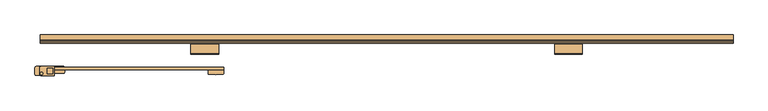
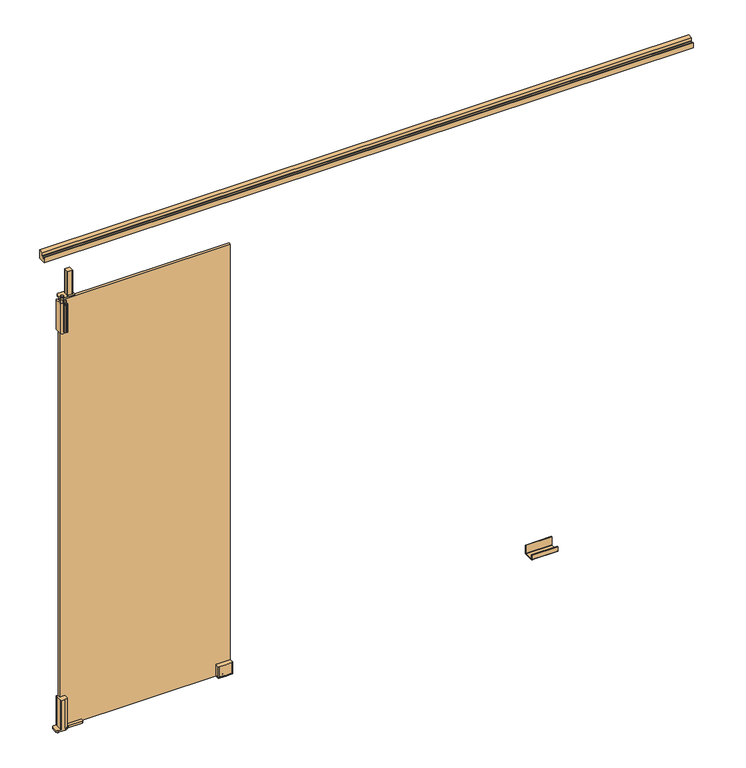
"""IFC4 building model written with IfcOpenShell, lengths in millimetres: door geometry, Otomatik Kapı-Çift Kanat : Otomatik Kapı - Çift Kanat - 150-220."""

from ifc_helpers import new_model, si_unit, point, frame, frame_2d, origin, origin_with_axes, place, context, project, spatial, polyline, circle_curve, trimmed, segment, composite_curve, outline, extrude, source, transform, mapped, element, save
from ifc_brep_helpers import plane_surface, cylinder_surface, revolved_surface, advanced_brep


def door_c3ca8d1c(model_context):
    return source(origin(), model_context, "Body", "SolidModel", [
        advanced_brep(
        [(-1467.3535836, -45.0, 150.5), (-1467.3535836, -42.932554, 150.5), (-1469.2861376, -41.0, 150.5), (-1498.067446, -41.0, 150.5), (-1500.0, -42.932554, 150.5), (-1500.0, -78.2162961, 150.5), (-1498.2162961, -80.0, 150.5), (-1480.406782, -80.0, 150.5), (-1468.0, -73.2159914, 150.5), (-1468.0, -54.9832441, 150.5), (-1493.0, -54.9832441, 150.5), (-1493.0, -45.0, 150.5), (-1471.9265924, -76.964766, 8.0), (-1470.1692976, -75.2261826, 8.0), (-1468.0, -73.2159914, 8.0), (-1493.0, -45.0, 8.0), (-1467.3535836, -45.0, 8.0), (-1493.0, -54.9832441, 8.0), (-1468.0, -54.9832441, 8.0), (-1480.406782, -80.0, 8.0), (-1498.2162961, -80.0, 8.0), (-1512.8478933, -80.0, 8.0), (-1512.8478933, -80.0, 0.0), (-1480.406782, -80.0, 0.0), (-1500.0, -78.2162961, 8.0), (-1500.0, -42.932554, 8.0), (-1498.067446, -41.0, 8.0), (-1469.2861376, -41.0, 8.0), (-1397.0062198, -41.0, 8.0), (-1397.0062198, -41.0, 0.0), (-1512.9502869, -41.0, 0.0), (-1512.9502869, -41.0, 8.0), (-1467.3535836, -42.932554, 8.0), (-1392.0062198, -46.0, 0.0), (-1392.0062198, -66.0, 0.0), (-1397.0062198, -71.0, 0.0), (-1461.1062198, -71.0, 0.0), (-1470.1692976, -75.2261826, 0.0), (-1520.0062198, -72.8416735, 0.0), (-1520.0062198, -48.0559329, 0.0), (-1520.0062198, -48.0559329, 8.0), (-1520.0062198, -72.8416735, 8.0), (-1461.1062198, -71.0, 8.0), (-1397.0062198, -71.0, 8.0), (-1392.0062198, -66.0, 8.0), (-1392.0062198, -46.0, 8.0)],
        [
            (0, 1),
            (1, 2, circle_curve(frame((-1469.2861376, -42.932554, 150.5), z_axis=(0.0, 0.0, 1.0), x_axis=(1.0, 0.0, 0.0)), 1.932554)),
            (2, 3),
            (3, 4, circle_curve(frame((-1498.067446, -42.932554, 150.5), z_axis=(0.0, 0.0, 1.0), x_axis=(1.0, 0.0, 0.0)), 1.932554)),
            (4, 5),
            (5, 6, circle_curve(frame((-1498.2162961, -78.2162961, 150.5), z_axis=(0.0, 0.0, 1.0), x_axis=(1.0, 0.0, 0.0)), 1.7837039)),
            (6, 7),
            (7, 8, circle_curve(frame((-1481.829294, -62.6615339, 150.5), z_axis=(0.0, 0.0, 1.0), x_axis=(1.0, 0.0, 0.0)), 17.3967223)),
            (8, 9),
            (9, 10),
            (10, 11),
            (11, 0),
            (12, 13, circle_curve(frame((-1480.406782, -66.6359132, 8.0), z_axis=(0.0, 0.0, 1.0), x_axis=(1.0, 0.0, 0.0)), 13.3640868)),
            (13, 14, circle_curve(frame((-1461.1062198, -82.8310079, 8.0), z_axis=(0.0, 0.0, -1.0), x_axis=(1.0, 0.0, 0.0)), 11.8310079)),
            (14, 12, circle_curve(frame((-1481.829294, -62.6615339, 8.0), z_axis=(0.0, 0.0, -1.0), x_axis=(1.0, 0.0, 0.0)), 17.3967223)),
            (11, 15),
            (15, 16),
            (16, 0),
            (10, 17),
            (17, 15),
            (9, 18),
            (18, 17),
            (8, 14),
            (14, 18),
            (7, 19),
            (19, 12, circle_curve(frame((-1481.829294, -62.6615339, 8.0), z_axis=(0.0, 0.0, 1.0), x_axis=(1.0, 0.0, 0.0)), 17.3967223)),
            (6, 20),
            (20, 21),
            (21, 22),
            (22, 23),
            (23, 19),
            (5, 24),
            (24, 20, circle_curve(frame((-1498.2162961, -78.2162961, 8.0), z_axis=(0.0, 0.0, 1.0), x_axis=(1.0, 0.0, 0.0)), 1.7837039)),
            (4, 25),
            (25, 24),
            (3, 26),
            (26, 25, circle_curve(frame((-1498.067446, -42.932554, 8.0), z_axis=(0.0, 0.0, 1.0), x_axis=(1.0, 0.0, 0.0)), 1.932554)),
            (2, 27),
            (27, 28),
            (28, 29),
            (29, 30),
            (30, 31),
            (31, 26),
            (1, 32),
            (32, 27, circle_curve(frame((-1469.2861376, -42.932554, 8.0), z_axis=(0.0, 0.0, 1.0), x_axis=(1.0, 0.0, 0.0)), 1.932554)),
            (16, 32),
            (29, 33, circle_curve(frame((-1397.0062198, -46.0, 0.0), z_axis=(0.0, 0.0, -1.0), x_axis=(1.0, 0.0, 0.0)), 5.0)),
            (33, 34),
            (34, 35, circle_curve(frame((-1397.0062198, -66.0, 0.0), z_axis=(0.0, 0.0, -1.0), x_axis=(1.0, 0.0, 0.0)), 5.0)),
            (35, 36),
            (36, 37, circle_curve(frame((-1461.1062198, -82.8310079, 0.0), z_axis=(0.0, 0.0, 1.0), x_axis=(1.0, 0.0, 0.0)), 11.8310079)),
            (37, 23, circle_curve(frame((-1480.406782, -66.6359132, 0.0), z_axis=(0.0, 0.0, -1.0), x_axis=(1.0, 0.0, 0.0)), 13.3640868)),
            (22, 38, circle_curve(frame((-1512.8478933, -72.8416735, 0.0), z_axis=(0.0, 0.0, -1.0), x_axis=(1.0, 0.0, 0.0)), 7.1583265)),
            (38, 39),
            (39, 30, circle_curve(frame((-1512.9502869, -48.0559329, 0.0), z_axis=(0.0, 0.0, -1.0), x_axis=(1.0, 0.0, 0.0)), 7.0559329)),
            (19, 12, circle_curve(frame((-1480.406782, -66.6359132, 8.0), z_axis=(0.0, 0.0, 1.0), x_axis=(1.0, 0.0, 0.0)), 13.3640868)),
            (31, 40, circle_curve(frame((-1512.9502869, -48.0559329, 8.0), z_axis=(0.0, 0.0, 1.0), x_axis=(1.0, 0.0, 0.0)), 7.0559329)),
            (40, 41),
            (41, 21, circle_curve(frame((-1512.8478933, -72.8416735, 8.0), z_axis=(0.0, 0.0, 1.0), x_axis=(1.0, 0.0, 0.0)), 7.1583265)),
            (14, 42, circle_curve(frame((-1461.1062198, -82.8310079, 8.0), z_axis=(0.0, 0.0, -1.0), x_axis=(1.0, 0.0, 0.0)), 11.8310079)),
            (42, 43),
            (43, 44, circle_curve(frame((-1397.0062198, -66.0, 8.0), z_axis=(0.0, 0.0, 1.0), x_axis=(1.0, 0.0, 0.0)), 5.0)),
            (44, 45),
            (45, 28, circle_curve(frame((-1397.0062198, -46.0, 8.0), z_axis=(0.0, 0.0, 1.0), x_axis=(1.0, 0.0, 0.0)), 5.0)),
            (39, 40),
            (38, 41),
            (37, 13),
            (36, 42),
            (35, 43),
            (34, 44),
            (33, 45),
        ],
        [
            plane_surface(frame((-1520.0062198, -41.0, 150.5), z_axis=(0.0, 0.0, 1.0), x_axis=(0.0, 1.0, 0.0))),
            plane_surface(frame((-1520.0062198, -41.0, 8.0), z_axis=(0.0, 0.0, -1.0), x_axis=(0.0, 1.0, 0.0))),
            plane_surface(frame((-1467.3535836, -45.0, 150.5), z_axis=(0.0, -1.0, 0.0), x_axis=(0.0, 0.0, -1.0))),
            plane_surface(frame((-1493.0, -45.0, 150.5), z_axis=(1.0, 0.0, 0.0), x_axis=(0.0, 0.0, -1.0))),
            plane_surface(frame((-1493.0, -54.9832441, 150.5), z_axis=(0.0, 1.0, 0.0), x_axis=(0.0, 0.0, -1.0))),
            plane_surface(frame((-1468.0, -54.9832441, 150.5), z_axis=(1.0, 0.0, 0.0), x_axis=(0.0, 0.0, -1.0))),
            cylinder_surface(frame((-1481.829294, -62.6615339, 150.5), z_axis=(0.0, 0.0, 1.0), x_axis=(1.0, 0.0, 0.0)), 17.3967223),
            plane_surface(frame((-1480.406782, -80.0, 150.5), z_axis=(0.0, -1.0, 0.0), x_axis=(0.0, 0.0, -1.0))),
            cylinder_surface(frame((-1498.2162961, -78.2162961, 150.5), z_axis=(0.0, 0.0, 1.0), x_axis=(1.0, 0.0, 0.0)), 1.7837039),
            plane_surface(frame((-1500.0, -78.2162961, 150.5), z_axis=(-1.0, 0.0, 0.0), x_axis=(0.0, 0.0, -1.0))),
            cylinder_surface(frame((-1498.067446, -42.932554, 150.5), z_axis=(0.0, 0.0, 1.0), x_axis=(1.0, 0.0, 0.0)), 1.932554),
            plane_surface(frame((-1498.067446, -41.0, 150.5), z_axis=(0.0, 1.0, 0.0), x_axis=(0.0, 0.0, -1.0))),
            cylinder_surface(frame((-1469.2861376, -42.932554, 150.5), z_axis=(0.0, 0.0, 1.0), x_axis=(1.0, 0.0, 0.0)), 1.932554),
            plane_surface(frame((-1467.3535836, -42.932554, 150.5), z_axis=(1.0, 0.0, 0.0), x_axis=(0.0, 0.0, -1.0))),
            plane_surface(frame((-1520.0062198, -41.0, 0.0), z_axis=(0.0, 0.0, -1.0), x_axis=(0.0, 1.0, 0.0))),
            plane_surface(frame((-1520.0062198, -41.0, 8.0), z_axis=(0.0, 0.0, 1.0), x_axis=(0.0, 1.0, 0.0))),
            cylinder_surface(frame((-1512.9502869, -48.0559329, 0.0), z_axis=(0.0, 0.0, -1.0), x_axis=(1.0, 0.0, 0.0)), 7.0559329),
            plane_surface(frame((-1520.0062198, -48.0559329, 0.0), z_axis=(-1.0, 0.0, 0.0), x_axis=(0.0, 0.0, 1.0))),
            cylinder_surface(frame((-1512.8478933, -72.8416735, 0.0), z_axis=(0.0, 0.0, -1.0), x_axis=(1.0, 0.0, 0.0)), 7.1583265),
            cylinder_surface(frame((-1480.406782, -66.6359132, 0.0), z_axis=(0.0, 0.0, -1.0), x_axis=(1.0, 0.0, 0.0)), 13.3640868),
            revolved_surface(polyline([(-1449.2752119, -82.8310079, 8.0), (-1449.2752119, -82.8310079, 0.0)]), (-1461.1062198, -82.8310079, 0.0), (0.0, 0.0, 1.0)),
            plane_surface(frame((-1461.1062198, -71.0, 0.0), z_axis=(0.0, -1.0, 0.0), x_axis=(0.0, 0.0, 1.0))),
            cylinder_surface(frame((-1397.0062198, -66.0, 0.0), z_axis=(0.0, 0.0, -1.0), x_axis=(1.0, 0.0, 0.0)), 5.0),
            plane_surface(frame((-1392.0062198, -66.0, 0.0), z_axis=(1.0, 0.0, 0.0), x_axis=(0.0, 0.0, 1.0))),
            cylinder_surface(frame((-1397.0062198, -46.0, 0.0), z_axis=(0.0, 0.0, -1.0), x_axis=(1.0, 0.0, 0.0)), 5.0),
        ],
        [
            (0, [[1, 2, 3, 4, 5, 6, 7, 8, 9, 10, 11, 12]]),
            (1, [[13, 14, 15]]),
            (2, [[16, 17, 18, -12]]),
            (3, [[19, 20, -16, -11]]),
            (4, [[21, 22, -19, -10]]),
            (5, [[23, 24, -21, -9]]),
            (6, [[25, 26, -15, -23, -8]]),
            (7, [[27, 28, 29, 30, 31, -25, -7]]),
            (8, [[32, 33, -27, -6]]),
            (9, [[34, 35, -32, -5]]),
            (10, [[36, 37, -34, -4]]),
            (11, [[38, 39, 40, 41, 42, 43, -36, -3]]),
            (12, [[44, 45, -38, -2]]),
            (13, [[-18, 46, -44, -1]]),
            (14, [[47, 48, 49, 50, 51, 52, -30, 53, 54, 55, -41]]),
            (15, [[-26, 56]]),
            (15, [[-28, -33, -35, -37, -43, 57, 58, 59]]),
            (15, [[-39, -45, -46, -17, -20, -22, -24, 60, 61, 62, 63, 64]]),
            (16, [[65, -57, -42, -55]]),
            (17, [[66, -58, -65, -54]]),
            (18, [[-29, -59, -66, -53]]),
            (19, [[67, -13, -56, -31, -52]]),
            (20, [[68, -60, -14, -67, -51]]),
            (21, [[69, -61, -68, -50]]),
            (22, [[70, -62, -69, -49]]),
            (23, [[71, -63, -70, -48]]),
            (24, [[-40, -64, -71, -47]]),
        ],
    ),
        advanced_brep(
        [(-1465.150075, -48.2790947, 2225.0), (-1466.9853602, -50.1143799, 2225.0), (-1466.9853602, -71.4438095, 2225.0), (-1465.150075, -73.2790947, 2225.0), (-1443.8206454, -73.2790947, 2225.0), (-1441.9853602, -71.4438095, 2225.0), (-1441.9853602, -50.1143799, 2225.0), (-1443.8206454, -48.2790947, 2225.0), (-1443.8206454, -48.2790947, 2110.0), (-1465.150075, -48.2790947, 2110.0), (-1441.9853602, -50.1143799, 2110.0), (-1441.9853602, -71.4438095, 2110.0), (-1443.8206454, -73.2790947, 2110.0), (-1465.150075, -73.2790947, 2110.0), (-1466.9853602, -71.4438095, 2110.0), (-1466.9853602, -50.1143799, 2110.0), (-1439.0026222, -41.0, 2110.0), (-1491.1711596, -41.0, 2110.0), (-1500.0, -49.8288404, 2110.0), (-1500.0, -72.0, 2110.0), (-1491.0, -81.0, 2110.0), (-1439.3215757, -81.0, 2110.0), (-1436.0, -77.6784243, 2110.0), (-1436.0, -44.0026222, 2110.0), (-1491.0, -77.9, 2110.0), (-1491.0, -66.1, 2110.0), (-1439.0026222, -41.0, 2104.0), (-1436.0, -44.0026222, 2104.0), (-1436.0, -77.6784243, 2104.0), (-1439.3215757, -81.0, 2104.0), (-1491.0, -81.0, 2104.0), (-1500.0, -72.0, 2104.0), (-1500.0, -49.8288404, 2104.0), (-1491.1711596, -41.0, 2104.0), (-1491.0, -66.1, 2104.0), (-1491.0, -77.9, 2104.0), (-1500.0, -72.0, 1938.2), (-1500.0, -42.2116006, 1938.2), (-1498.7883994, -41.0, 1938.2), (-1469.3259879, -41.0, 1938.2), (-1468.0, -42.3259879, 1938.2), (-1468.0, -45.1, 1938.2), (-1492.8, -45.1, 1938.2), (-1492.8, -55.1, 1938.2), (-1468.0, -55.1, 1938.2), (-1468.0, -77.9, 1938.2), (-1471.1, -81.0, 1938.2), (-1480.4177248, -81.0, 1938.2), (-1484.4524153, -78.1748793, 1938.2), (-1480.2256421, -66.1, 1938.2), (-1482.0, -67.8743579, 1938.2), (-1482.0, -75.7274684, 1938.2), (-1480.1735897, -77.9, 1938.2), (-1472.0887779, -77.9, 1938.2), (-1471.1, -76.9112221, 1938.2), (-1471.1, -66.1, 1938.2), (-1491.0, -66.1, 1938.2), (-1491.0, -77.9, 1938.2), (-1500.0, -72.0, 2083.2), (-1482.0, -72.0, 2083.2), (-1482.0, -67.8743579, 2083.2), (-1480.2256421, -66.1, 2083.2), (-1469.1779802, -66.1, 2083.2), (-1468.0, -64.9220198, 2083.2), (-1468.0, -55.1, 2083.2), (-1492.8, -55.1, 2083.2), (-1492.8, -45.1, 2083.2), (-1468.0, -45.1, 2083.2), (-1468.0, -42.3259879, 2083.2), (-1469.3259879, -41.0, 2083.2), (-1498.7883994, -41.0, 2083.2), (-1500.0, -42.2116006, 2083.2), (-1491.0, -77.9, 2083.2), (-1491.0, -66.1, 2083.2), (-1468.0, -64.9220198, 2073.2), (-1468.0, -77.9, 2073.2), (-1469.1779802, -66.1, 2073.2), (-1471.1, -66.1, 2073.2), (-1482.0, -72.0, 2073.2), (-1482.0, -75.7274684, 2073.2), (-1484.4524153, -78.1748793, 2073.2), (-1491.0, -66.1, 2083.2), (-1491.0, -77.9, 2083.2), (-1471.1, -81.0, 2073.2), (-1471.1, -76.9112221, 2073.2), (-1472.0887779, -77.9, 2073.2), (-1480.1735897, -77.9, 2073.2), (-1480.4177248, -81.0, 2073.2), (-1491.0, -66.1, 2116.5286826), (-1491.0, -77.9, 2116.5286826)],
        [
            (0, 1, circle_curve(frame((-1465.150075, -50.1143799, 2225.0), z_axis=(0.0, 0.0, 1.0), x_axis=(0.0, -1.0, 0.0)), 1.8352852)),
            (1, 2),
            (2, 3, circle_curve(frame((-1465.150075, -71.4438095, 2225.0), z_axis=(0.0, 0.0, 1.0), x_axis=(0.0, 1.0, 0.0)), 1.8352852)),
            (3, 4),
            (4, 5, circle_curve(frame((-1443.8206454, -71.4438095, 2225.0), z_axis=(0.0, 0.0, 1.0), x_axis=(0.0, 1.0, 0.0)), 1.8352852)),
            (5, 6),
            (6, 7, circle_curve(frame((-1443.8206454, -50.1143799, 2225.0), z_axis=(0.0, 0.0, 1.0), x_axis=(0.0, -1.0, 0.0)), 1.8352852)),
            (7, 0),
            (7, 8),
            (8, 9),
            (9, 0),
            (6, 10),
            (10, 8, circle_curve(frame((-1443.8206454, -50.1143799, 2110.0), z_axis=(0.0, 0.0, 1.0), x_axis=(0.0, -1.0, 0.0)), 1.8352852)),
            (5, 11),
            (11, 10),
            (4, 12),
            (12, 11, circle_curve(frame((-1443.8206454, -71.4438095, 2110.0), z_axis=(0.0, 0.0, 1.0), x_axis=(0.0, 1.0, 0.0)), 1.8352852)),
            (3, 13),
            (13, 12),
            (2, 14),
            (14, 13, circle_curve(frame((-1465.150075, -71.4438095, 2110.0), z_axis=(0.0, 0.0, 1.0), x_axis=(0.0, 1.0, 0.0)), 1.8352852)),
            (1, 15),
            (15, 14),
            (9, 15, circle_curve(frame((-1465.150075, -50.1143799, 2110.0), z_axis=(0.0, 0.0, 1.0), x_axis=(0.0, -1.0, 0.0)), 1.8352852)),
            (16, 17),
            (17, 18, circle_curve(frame((-1491.1711596, -49.8288404, 2110.0), z_axis=(0.0, 0.0, 1.0), x_axis=(0.0, -1.0, 0.0)), 8.8288404)),
            (18, 19),
            (19, 20, circle_curve(frame((-1491.0, -72.0, 2110.0), z_axis=(0.0, 0.0, 1.0), x_axis=(0.0, -1.0, 0.0)), 9.0)),
            (20, 21),
            (21, 22, circle_curve(frame((-1439.3215757, -77.6784243, 2110.0), z_axis=(0.0, 0.0, 1.0), x_axis=(0.0, -1.0, 0.0)), 3.3215757)),
            (22, 23),
            (23, 16, circle_curve(frame((-1439.0026222, -44.0026222, 2110.0), z_axis=(0.0, 0.0, 1.0), x_axis=(0.0, -1.0, 0.0)), 3.0026222)),
            (24, 25, circle_curve(frame((-1491.0, -72.0, 2110.0), z_axis=(0.0, 0.0, -1.0), x_axis=(0.0, -1.0, 0.0)), 5.9)),
            (25, 24, circle_curve(frame((-1491.0, -72.0, 2110.0), z_axis=(0.0, 0.0, -1.0), x_axis=(0.0, -1.0, 0.0)), 5.9)),
            (26, 27, circle_curve(frame((-1439.0026222, -44.0026222, 2104.0), z_axis=(0.0, 0.0, -1.0), x_axis=(0.0, -1.0, 0.0)), 3.0026222)),
            (27, 28),
            (28, 29, circle_curve(frame((-1439.3215757, -77.6784243, 2104.0), z_axis=(0.0, 0.0, -1.0), x_axis=(0.0, -1.0, 0.0)), 3.3215757)),
            (29, 30),
            (30, 31, circle_curve(frame((-1491.0, -72.0, 2104.0), z_axis=(0.0, 0.0, -1.0), x_axis=(0.0, -1.0, 0.0)), 9.0)),
            (31, 32),
            (32, 33, circle_curve(frame((-1491.1711596, -49.8288404, 2104.0), z_axis=(0.0, 0.0, -1.0), x_axis=(0.0, -1.0, 0.0)), 8.8288404)),
            (33, 26),
            (34, 35, circle_curve(frame((-1491.0, -72.0, 2104.0), z_axis=(0.0, 0.0, 1.0), x_axis=(0.0, -1.0, 0.0)), 5.9)),
            (35, 34, circle_curve(frame((-1491.0, -72.0, 2104.0), z_axis=(0.0, 0.0, 1.0), x_axis=(0.0, -1.0, 0.0)), 5.9)),
            (16, 26),
            (33, 17),
            (32, 18),
            (31, 19),
            (30, 20),
            (29, 21),
            (28, 22),
            (27, 23),
            (36, 37),
            (37, 38, circle_curve(frame((-1498.7883994, -42.2116006, 1938.2), z_axis=(0.0, 0.0, -1.0), x_axis=(0.0, -1.0, 0.0)), 1.2116006)),
            (38, 39),
            (39, 40, circle_curve(frame((-1469.3259879, -42.3259879, 1938.2), z_axis=(0.0, 0.0, -1.0), x_axis=(0.0, -1.0, 0.0)), 1.3259879)),
            (40, 41),
            (41, 42),
            (42, 43),
            (43, 44),
            (44, 45),
            (45, 46, circle_curve(frame((-1471.1, -77.9, 1938.2), z_axis=(0.0, 0.0, -1.0), x_axis=(0.0, -1.0, 0.0)), 3.1)),
            (46, 47),
            (47, 48, circle_curve(frame((-1479.7322891, -75.7274684, 1938.2), z_axis=(0.0, 0.0, -1.0), x_axis=(0.0, -1.0, 0.0)), 5.3168987)),
            (48, 36, circle_curve(frame((-1491.0, -72.0, 1938.2), z_axis=(0.0, 0.0, -1.0), x_axis=(0.0, -1.0, 0.0)), 9.0)),
            (49, 50, circle_curve(frame((-1480.2256421, -67.8743579, 1938.2), z_axis=(0.0, 0.0, 1.0), x_axis=(0.0, -1.0, 0.0)), 1.7743579)),
            (50, 51),
            (51, 52, circle_curve(frame((-1479.7322891, -75.7274684, 1938.2), z_axis=(0.0, 0.0, 1.0), x_axis=(0.0, -1.0, 0.0)), 2.2168987)),
            (52, 53),
            (53, 54, circle_curve(frame((-1472.0887779, -76.9112221, 1938.2), z_axis=(0.0, 0.0, 1.0), x_axis=(0.0, -1.0, 0.0)), 0.9887779)),
            (54, 55),
            (55, 49),
            (56, 57, circle_curve(frame((-1491.0, -72.0, 1938.2), z_axis=(0.0, 0.0, 1.0), x_axis=(0.0, -1.0, 0.0)), 5.9)),
            (57, 56, circle_curve(frame((-1491.0, -72.0, 1938.2), z_axis=(0.0, 0.0, 1.0), x_axis=(0.0, -1.0, 0.0)), 5.9)),
            (58, 59, circle_curve(frame((-1491.0, -72.0, 2083.2), z_axis=(0.0, 0.0, 1.0), x_axis=(0.0, -1.0, 0.0)), 9.0)),
            (59, 60),
            (60, 61, circle_curve(frame((-1480.2256421, -67.8743579, 2083.2), z_axis=(0.0, 0.0, -1.0), x_axis=(0.0, -1.0, 0.0)), 1.7743579)),
            (61, 62),
            (62, 63, circle_curve(frame((-1469.1779802, -64.9220198, 2083.2), z_axis=(0.0, 0.0, 1.0), x_axis=(0.0, -1.0, 0.0)), 1.1779802)),
            (63, 64),
            (64, 65),
            (65, 66),
            (66, 67),
            (67, 68),
            (68, 69, circle_curve(frame((-1469.3259879, -42.3259879, 2083.2), z_axis=(0.0, 0.0, 1.0), x_axis=(0.0, -1.0, 0.0)), 1.3259879)),
            (69, 70),
            (70, 71, circle_curve(frame((-1498.7883994, -42.2116006, 2083.2), z_axis=(0.0, 0.0, 1.0), x_axis=(0.0, -1.0, 0.0)), 1.2116006)),
            (71, 58),
            (72, 73, circle_curve(frame((-1491.0, -72.0, 2083.2), z_axis=(0.0, 0.0, -1.0), x_axis=(0.0, -1.0, 0.0)), 5.9)),
            (73, 72, circle_curve(frame((-1491.0, -72.0, 2083.2), z_axis=(0.0, 0.0, -1.0), x_axis=(0.0, -1.0, 0.0)), 5.9)),
            (36, 58),
            (71, 37),
            (70, 38),
            (69, 39),
            (68, 40),
            (67, 41),
            (66, 42),
            (65, 43),
            (64, 44),
            (63, 74),
            (74, 75),
            (75, 45),
            (62, 76),
            (76, 74, circle_curve(frame((-1469.1779802, -64.9220198, 2073.2), z_axis=(0.0, 0.0, 1.0), x_axis=(0.0, -1.0, 0.0)), 1.1779802)),
            (61, 49),
            (55, 77),
            (77, 76),
            (60, 50),
            (59, 78),
            (78, 79),
            (79, 51),
            (48, 80),
            (80, 78, circle_curve(frame((-1491.0, -72.0, 2073.2), z_axis=(0.0, 0.0, 1.0), x_axis=(0.0, -1.0, 0.0)), 9.0)),
            (56, 81),
            (81, 82, circle_curve(frame((-1491.0, -72.0, 2083.2), z_axis=(0.0, 0.0, 1.0), x_axis=(0.0, -1.0, 0.0)), 5.9)),
            (82, 57),
            (82, 81, circle_curve(frame((-1491.0, -72.0, 2083.2), z_axis=(0.0, 0.0, 1.0), x_axis=(0.0, -1.0, 0.0)), 5.9)),
            (83, 75, circle_curve(frame((-1471.1, -77.9, 2073.2), z_axis=(0.0, 0.0, 1.0), x_axis=(0.0, -1.0, 0.0)), 3.1)),
            (77, 84),
            (84, 85, circle_curve(frame((-1472.0887779, -76.9112221, 2073.2), z_axis=(0.0, 0.0, -1.0), x_axis=(0.0, -1.0, 0.0)), 0.9887779)),
            (85, 86),
            (86, 79, circle_curve(frame((-1479.7322891, -75.7274684, 2073.2), z_axis=(0.0, 0.0, -1.0), x_axis=(0.0, -1.0, 0.0)), 2.2168987)),
            (80, 87, circle_curve(frame((-1479.7322891, -75.7274684, 2073.2), z_axis=(0.0, 0.0, 1.0), x_axis=(0.0, -1.0, 0.0)), 5.3168987)),
            (87, 83),
            (83, 46),
            (54, 84),
            (53, 85),
            (52, 86),
            (47, 87),
            (88, 89, circle_curve(frame((-1491.0, -72.0, 2116.5286826), z_axis=(0.0, 0.0, 1.0), x_axis=(0.0, -1.0, 0.0)), 5.9)),
            (89, 88, circle_curve(frame((-1491.0, -72.0, 2116.5286826), z_axis=(0.0, 0.0, 1.0), x_axis=(0.0, -1.0, 0.0)), 5.9)),
            (88, 25),
            (24, 89),
            (34, 73),
            (72, 35),
        ],
        [
            plane_surface(frame((-1500.0, -41.0, 2225.0), z_axis=(0.0, 0.0, 1.0), x_axis=(-1.0, 0.0, 0.0))),
            plane_surface(frame((-1465.150075, -48.2790947, 2110.0), z_axis=(0.0, 1.0, 0.0), x_axis=(0.0, 0.0, 1.0))),
            cylinder_surface(frame((-1443.8206454, -50.1143799, 2110.0), z_axis=(0.0, 0.0, -1.0), x_axis=(0.0, -1.0, 0.0)), 1.8352852),
            plane_surface(frame((-1441.9853602, -50.1143799, 2110.0), z_axis=(1.0, 0.0, 0.0), x_axis=(0.0, 0.0, 1.0))),
            cylinder_surface(frame((-1443.8206454, -71.4438095, 2110.0), z_axis=(0.0, 0.0, -1.0), x_axis=(0.0, 1.0, 0.0)), 1.8352852),
            plane_surface(frame((-1443.8206454, -73.2790947, 2110.0), z_axis=(0.0, -1.0, 0.0), x_axis=(0.0, 0.0, 1.0))),
            cylinder_surface(frame((-1465.150075, -71.4438095, 2110.0), z_axis=(0.0, 0.0, -1.0), x_axis=(0.0, 1.0, 0.0)), 1.8352852),
            plane_surface(frame((-1466.9853602, -71.4438095, 2110.0), z_axis=(-1.0, 0.0, 0.0), x_axis=(0.0, 0.0, 1.0))),
            cylinder_surface(frame((-1465.150075, -50.1143799, 2110.0), z_axis=(0.0, 0.0, -1.0), x_axis=(0.0, -1.0, 0.0)), 1.8352852),
            plane_surface(frame((-1500.0, -41.0, 2110.0), z_axis=(0.0, 0.0, 1.0), x_axis=(-1.0, 0.0, 0.0))),
            plane_surface(frame((-1500.0, -41.0, 2104.0), z_axis=(0.0, 0.0, -1.0), x_axis=(-1.0, 0.0, 0.0))),
            plane_surface(frame((-1439.0026222, -41.0, 2110.0), z_axis=(0.0, 1.0, 0.0), x_axis=(0.0, 0.0, -1.0))),
            cylinder_surface(frame((-1491.1711596, -49.8288404, 2110.0), z_axis=(0.0, 0.0, 1.0), x_axis=(0.0, -1.0, 0.0)), 8.8288404),
            plane_surface(frame((-1500.0, -49.8288404, 2110.0), z_axis=(-1.0, 0.0, 0.0), x_axis=(0.0, 0.0, -1.0))),
            cylinder_surface(frame((-1491.0, -72.0, 2110.0), z_axis=(0.0, 0.0, 1.0), x_axis=(0.0, -1.0, 0.0)), 9.0),
            plane_surface(frame((-1491.0, -81.0, 2110.0), z_axis=(0.0, -1.0, 0.0), x_axis=(0.0, 0.0, -1.0))),
            cylinder_surface(frame((-1439.3215757, -77.6784243, 2110.0), z_axis=(0.0, 0.0, 1.0), x_axis=(0.0, -1.0, 0.0)), 3.3215757),
            plane_surface(frame((-1436.0, -77.6784243, 2110.0), z_axis=(1.0, 0.0, 0.0), x_axis=(0.0, 0.0, -1.0))),
            cylinder_surface(frame((-1439.0026222, -44.0026222, 2110.0), z_axis=(0.0, 0.0, 1.0), x_axis=(0.0, -1.0, 0.0)), 3.0026222),
            plane_surface(frame((-1500.0, -41.0, 1938.2), z_axis=(0.0, 0.0, -1.0), x_axis=(-1.0, 0.0, 0.0))),
            plane_surface(frame((-1500.0, -41.0, 2083.2), z_axis=(0.0, 0.0, 1.0), x_axis=(-1.0, 0.0, 0.0))),
            plane_surface(frame((-1500.0, -72.0, 1938.2), z_axis=(-1.0, 0.0, 0.0), x_axis=(0.0, 0.0, 1.0))),
            cylinder_surface(frame((-1498.7883994, -42.2116006, 1938.2), z_axis=(0.0, 0.0, -1.0), x_axis=(0.0, -1.0, 0.0)), 1.2116006),
            plane_surface(frame((-1498.7883994, -41.0, 1938.2), z_axis=(0.0, 1.0, 0.0), x_axis=(0.0, 0.0, 1.0))),
            cylinder_surface(frame((-1469.3259879, -42.3259879, 1938.2), z_axis=(0.0, 0.0, -1.0), x_axis=(0.0, -1.0, 0.0)), 1.3259879),
            plane_surface(frame((-1468.0, -42.3259879, 1938.2), z_axis=(1.0, 0.0, 0.0), x_axis=(0.0, 0.0, 1.0))),
            plane_surface(frame((-1468.0, -45.1, 1938.2), z_axis=(0.0, -1.0, 0.0), x_axis=(0.0, 0.0, 1.0))),
            plane_surface(frame((-1492.8, -45.1, 1938.2), z_axis=(1.0, 0.0, 0.0), x_axis=(0.0, 0.0, 1.0))),
            plane_surface(frame((-1492.8, -55.1, 1938.2), z_axis=(0.0, 1.0, 0.0), x_axis=(0.0, 0.0, 1.0))),
            plane_surface(frame((-1468.0, -55.1, 1938.2), z_axis=(1.0, 0.0, 0.0), x_axis=(0.0, 0.0, 1.0))),
            cylinder_surface(frame((-1469.1779802, -64.9220198, 1938.2), z_axis=(0.0, 0.0, -1.0), x_axis=(0.0, -1.0, 0.0)), 1.1779802),
            plane_surface(frame((-1469.1779802, -66.1, 1938.2), z_axis=(0.0, -1.0, 0.0), x_axis=(0.0, 0.0, 1.0))),
            revolved_surface(polyline([(-1480.2256421, -69.6487158, 2083.2), (-1480.2256421, -69.6487158, 1938.2)]), (-1480.2256421, -67.8743579, 1938.2), (0.0, 0.0, 1.0)),
            plane_surface(frame((-1482.0, -67.8743579, 1938.2), z_axis=(1.0, 0.0, 0.0), x_axis=(0.0, 0.0, 1.0))),
            cylinder_surface(frame((-1491.0, -72.0, 1938.2), z_axis=(0.0, 0.0, -1.0), x_axis=(0.0, -1.0, 0.0)), 9.0),
            revolved_surface(polyline([(-1491.0, -77.9, 2083.2), (-1491.0, -77.9, 1938.2)]), (-1491.0, -72.0, 1938.2), (0.0, 0.0, 1.0)),
            plane_surface(frame((-1500.0, -41.0, 2073.2), z_axis=(0.0, 0.0, 1.0), x_axis=(-1.0, 0.0, 0.0))),
            cylinder_surface(frame((-1471.1, -77.9, 2073.2), z_axis=(0.0, 0.0, 1.0), x_axis=(0.0, -1.0, 0.0)), 3.1),
            plane_surface(frame((-1471.1, -66.1, 2073.2), z_axis=(-1.0, 0.0, 0.0), x_axis=(0.0, 0.0, -1.0))),
            revolved_surface(polyline([(-1472.0887779, -77.9, 1938.2), (-1472.0887779, -77.9, 2073.2)]), (-1472.0887779, -76.9112221, 2073.2), (0.0, 0.0, -1.0)),
            plane_surface(frame((-1472.0887779, -77.9, 2073.2), z_axis=(0.0, 1.0, 0.0), x_axis=(0.0, 0.0, -1.0))),
            revolved_surface(polyline([(-1479.7322891, -77.94436710000001, 1938.2), (-1479.7322891, -77.94436710000001, 2073.2)]), (-1479.7322891, -75.7274684, 2073.2), (0.0, 0.0, -1.0)),
            cylinder_surface(frame((-1479.7322891, -75.7274684, 2073.2), z_axis=(0.0, 0.0, 1.0), x_axis=(0.0, -1.0, 0.0)), 5.3168987),
            plane_surface(frame((-1480.4177248, -81.0, 2073.2), z_axis=(0.0, -1.0, 0.0), x_axis=(0.0, 0.0, -1.0))),
            plane_surface(frame((-1500.0, -41.0, 2116.5286826), z_axis=(0.0, 0.0, 1.0), x_axis=(-1.0, 0.0, 0.0))),
            plane_surface(frame((-1500.0, -41.0, 2083.2), z_axis=(0.0, 0.0, -1.0), x_axis=(-1.0, 0.0, 0.0))),
            cylinder_surface(frame((-1491.0, -72.0, 2116.5286826), z_axis=(0.0, 0.0, 1.0), x_axis=(0.0, -1.0, 0.0)), 5.9),
        ],
        [
            (0, [[1, 2, 3, 4, 5, 6, 7, 8]]),
            (1, [[-8, 9, 10, 11]]),
            (2, [[-7, 12, 13, -9]]),
            (3, [[-6, 14, 15, -12]]),
            (4, [[-5, 16, 17, -14]]),
            (5, [[-4, 18, 19, -16]]),
            (6, [[-3, 20, 21, -18]]),
            (7, [[-2, 22, 23, -20]]),
            (8, [[-1, -11, 24, -22]]),
            (9, [[25, 26, 27, 28, 29, 30, 31, 32], [-10, -13, -15, -17, -19, -21, -23, -24], [33, 34]]),
            (10, [[35, 36, 37, 38, 39, 40, 41, 42], [43, 44]]),
            (11, [[-25, 45, -42, 46]]),
            (12, [[-26, -46, -41, 47]]),
            (13, [[-27, -47, -40, 48]]),
            (14, [[-28, -48, -39, 49]]),
            (15, [[-29, -49, -38, 50]]),
            (16, [[-30, -50, -37, 51]]),
            (17, [[-31, -51, -36, 52]]),
            (18, [[-32, -52, -35, -45]]),
            (19, [[53, 54, 55, 56, 57, 58, 59, 60, 61, 62, 63, 64, 65], [66, 67, 68, 69, 70, 71, 72], [73, 74]]),
            (20, [[75, 76, 77, 78, 79, 80, 81, 82, 83, 84, 85, 86, 87, 88], [89, 90]]),
            (21, [[-53, 91, -88, 92]]),
            (22, [[-54, -92, -87, 93]]),
            (23, [[-55, -93, -86, 94]]),
            (24, [[-56, -94, -85, 95]]),
            (25, [[-57, -95, -84, 96]]),
            (26, [[-58, -96, -83, 97]]),
            (27, [[-59, -97, -82, 98]]),
            (28, [[-60, -98, -81, 99]]),
            (29, [[-80, 100, 101, 102, -61, -99]]),
            (30, [[-79, 103, 104, -100]]),
            (31, [[-78, 105, -72, 106, 107, -103]]),
            (32, [[-66, -105, -77, 108]]),
            (33, [[-76, 109, 110, 111, -67, -108]]),
            (34, [[-75, -91, -65, 112, 113, -109]]),
            (35, [[-73, 114, 115, 116]]),
            (35, [[-74, -116, 117, -114]]),
            (36, [[118, -101, -104, -107, 119, 120, 121, 122, -110, -113, 123, 124]]),
            (37, [[-118, 125, -62, -102]]),
            (38, [[-119, -106, -71, 126]]),
            (39, [[-120, -126, -70, 127]]),
            (40, [[-121, -127, -69, 128]]),
            (41, [[-122, -128, -68, -111]]),
            (42, [[-123, -112, -64, 129]]),
            (43, [[-124, -129, -63, -125]]),
            (44, [[130, 131]]),
            (45, [[-115, -117]]),
            (46, [[-130, 132, -33, 133]]),
            (46, [[134, -89, 135, -43]]),
            (46, [[-131, -133, -34, -132]]),
            (46, [[-134, -44, -135, -90]]),
        ],
    ),
        advanced_brep(
        [(-768.5768027, -74.4811577, 6.5), (-770.8062198, -72.2517407, 6.5), (-770.8062198, -57.2607782, 6.5), (-768.5454415, -55.0, 6.5), (-707.066998, -55.0, 6.5), (-704.8062198, -57.2607782, 6.5), (-704.8062198, -72.2517407, 6.5), (-707.0356368, -74.4811577, 6.5), (-734.9062198, -59.6562595, 6.5), (-740.7062198, -59.6562595, 6.5), (-740.7062198, -69.8562595, 6.5), (-734.9062198, -69.8562595, 6.5), (-768.5768027, -74.4811577, 56.5), (-707.0356368, -74.4811577, 56.5), (-704.8062198, -72.2517407, 56.5), (-704.8062198, -57.2607782, 56.5), (-707.066998, -55.0, 56.5), (-768.5454415, -55.0, 56.5), (-770.8062198, -57.2607782, 56.5), (-770.8062198, -72.2517407, 56.5), (-734.9062198, -59.6562595, 4.0), (-740.7062198, -59.6562595, 4.0), (-740.7062198, -69.8562595, 4.0), (-734.9062198, -69.8562595, 4.0), (-768.5454415, -55.0, 0.0), (-707.066998, -55.0, 0.0), (-704.8062198, -57.2607782, 0.0), (-704.8062198, -72.2517407, 0.0), (-707.0356368, -74.4811577, 0.0), (-768.5768027, -74.4811577, 0.0), (-770.8062198, -72.2517407, 0.0), (-770.8062198, -57.2607782, 0.0), (-768.5454415, -55.0, 4.0), (-770.8062198, -57.2607782, 4.0), (-770.8062198, -72.2517407, 4.0), (-768.5768027, -74.4811577, 4.0), (-707.0356368, -74.4811577, 4.0), (-704.8062198, -72.2517407, 4.0), (-704.8062198, -57.2607782, 4.0), (-707.066998, -55.0, 4.0)],
        [
            (0, 1, circle_curve(frame((-767.1193692, -70.7943072, 6.5), z_axis=(0.0, 0.0, -1.0), x_axis=(-1.0, 0.0, 0.0)), 3.9644646)),
            (1, 2),
            (2, 3, circle_curve(frame((-768.5454415, -57.2607782, 6.5), z_axis=(0.0, 0.0, -1.0), x_axis=(1.0, 0.0, 0.0)), 2.2607782)),
            (3, 4),
            (4, 5, circle_curve(frame((-707.066998, -57.2607782, 6.5), z_axis=(0.0, 0.0, -1.0), x_axis=(-1.0, 0.0, 0.0)), 2.2607782)),
            (5, 6),
            (6, 7, circle_curve(frame((-708.4930703, -70.7943072, 6.5), z_axis=(0.0, 0.0, -1.0), x_axis=(1.0, 0.0, 0.0)), 3.9644646)),
            (7, 0, circle_curve(frame((-737.8062198, 112.2086207, 6.5), z_axis=(0.0, 0.0, -1.0), x_axis=(-1.0, 0.0, 0.0)), 189.2086207)),
            (8, 9),
            (9, 10, circle_curve(frame((-740.7062198, -64.7562595, 6.5), z_axis=(0.0, 0.0, 1.0), x_axis=(-1.0, 0.0, 0.0)), 5.1)),
            (10, 11),
            (11, 8, circle_curve(frame((-734.9062198, -64.7562595, 6.5), z_axis=(0.0, 0.0, 1.0), x_axis=(-1.0, 0.0, 0.0)), 5.1)),
            (12, 13, circle_curve(frame((-737.8062198, 112.2086207, 56.5), z_axis=(0.0, 0.0, 1.0), x_axis=(-1.0, 0.0, 0.0)), 189.2086207)),
            (13, 14, circle_curve(frame((-708.4930703, -70.7943072, 56.5), z_axis=(0.0, 0.0, 1.0), x_axis=(1.0, 0.0, 0.0)), 3.9644646)),
            (14, 15),
            (15, 16, circle_curve(frame((-707.066998, -57.2607782, 56.5), z_axis=(0.0, 0.0, 1.0), x_axis=(-1.0, 0.0, 0.0)), 2.2607782)),
            (16, 17),
            (17, 18, circle_curve(frame((-768.5454415, -57.2607782, 56.5), z_axis=(0.0, 0.0, 1.0), x_axis=(1.0, 0.0, 0.0)), 2.2607782)),
            (18, 19),
            (19, 12, circle_curve(frame((-767.1193692, -70.7943072, 56.5), z_axis=(0.0, 0.0, 1.0), x_axis=(-1.0, 0.0, 0.0)), 3.9644646)),
            (0, 12),
            (19, 1),
            (18, 2),
            (17, 3),
            (16, 4),
            (15, 5),
            (14, 6),
            (13, 7),
            (8, 20),
            (20, 21),
            (21, 9),
            (21, 22, circle_curve(frame((-740.7062198, -64.7562595, 4.0), z_axis=(0.0, 0.0, 1.0), x_axis=(-1.0, 0.0, 0.0)), 5.1)),
            (22, 10),
            (22, 23),
            (23, 11),
            (23, 20, circle_curve(frame((-734.9062198, -64.7562595, 4.0), z_axis=(0.0, 0.0, 1.0), x_axis=(-1.0, 0.0, 0.0)), 5.1)),
            (24, 25),
            (25, 26, circle_curve(frame((-707.066998, -57.2607782, 0.0), z_axis=(0.0, 0.0, -1.0), x_axis=(-1.0, 0.0, 0.0)), 2.2607782)),
            (26, 27),
            (27, 28, circle_curve(frame((-708.4930703, -70.7943072, 0.0), z_axis=(0.0, 0.0, -1.0), x_axis=(1.0, 0.0, 0.0)), 3.9644646)),
            (28, 29, circle_curve(frame((-737.8062198, 112.2086207, 0.0), z_axis=(0.0, 0.0, -1.0), x_axis=(-1.0, 0.0, 0.0)), 189.2086207)),
            (29, 30, circle_curve(frame((-767.1193692, -70.7943072, 0.0), z_axis=(0.0, 0.0, -1.0), x_axis=(-1.0, 0.0, 0.0)), 3.9644646)),
            (30, 31),
            (31, 24, circle_curve(frame((-768.5454415, -57.2607782, 0.0), z_axis=(0.0, 0.0, -1.0), x_axis=(1.0, 0.0, 0.0)), 2.2607782)),
            (32, 33, circle_curve(frame((-768.5454415, -57.2607782, 4.0), z_axis=(0.0, 0.0, 1.0), x_axis=(1.0, 0.0, 0.0)), 2.2607782)),
            (33, 34),
            (34, 35, circle_curve(frame((-767.1193692, -70.7943072, 4.0), z_axis=(0.0, 0.0, 1.0), x_axis=(-1.0, 0.0, 0.0)), 3.9644646)),
            (35, 36, circle_curve(frame((-737.8062198, 112.2086207, 4.0), z_axis=(0.0, 0.0, 1.0), x_axis=(-1.0, 0.0, 0.0)), 189.2086207)),
            (36, 37, circle_curve(frame((-708.4930703, -70.7943072, 4.0), z_axis=(0.0, 0.0, 1.0), x_axis=(1.0, 0.0, 0.0)), 3.9644646)),
            (37, 38),
            (38, 39, circle_curve(frame((-707.066998, -57.2607782, 4.0), z_axis=(0.0, 0.0, 1.0), x_axis=(-1.0, 0.0, 0.0)), 2.2607782)),
            (39, 32),
            (24, 32),
            (39, 25),
            (38, 26),
            (37, 27),
            (36, 28),
            (35, 29),
            (34, 30),
            (33, 31),
        ],
        [
            plane_surface(frame((-704.8062198, -55.0, 6.5), z_axis=(0.0, 0.0, -1.0), x_axis=(0.0, 1.0, 0.0))),
            plane_surface(frame((-704.8062198, -55.0, 56.5), z_axis=(0.0, 0.0, 1.0), x_axis=(0.0, 1.0, 0.0))),
            cylinder_surface(frame((-767.1193692, -70.7943072, 6.5), z_axis=(0.0, 0.0, -1.0), x_axis=(-1.0, 0.0, 0.0)), 3.9644646),
            plane_surface(frame((-770.8062198, -72.2517407, 6.5), z_axis=(-1.0, 0.0, 0.0), x_axis=(0.0, 0.0, 1.0))),
            cylinder_surface(frame((-768.5454415, -57.2607782, 6.5), z_axis=(0.0, 0.0, -1.0), x_axis=(1.0, 0.0, 0.0)), 2.2607782),
            plane_surface(frame((-768.5454415, -55.0, 6.5), z_axis=(0.0, 1.0, 0.0), x_axis=(0.0, 0.0, 1.0))),
            cylinder_surface(frame((-707.066998, -57.2607782, 6.5), z_axis=(0.0, 0.0, -1.0), x_axis=(-1.0, 0.0, 0.0)), 2.2607782),
            plane_surface(frame((-704.8062198, -57.2607782, 6.5), z_axis=(1.0, 0.0, 0.0), x_axis=(0.0, 0.0, 1.0))),
            cylinder_surface(frame((-708.4930703, -70.7943072, 6.5), z_axis=(0.0, 0.0, -1.0), x_axis=(1.0, 0.0, 0.0)), 3.9644646),
            cylinder_surface(frame((-737.8062198, 112.2086207, 6.5), z_axis=(0.0, 0.0, -1.0), x_axis=(-1.0, 0.0, 0.0)), 189.2086207),
            plane_surface(frame((-734.9062198, -59.6562595, 6.5), z_axis=(0.0, 1.0, 0.0), x_axis=(0.0, 0.0, -1.0))),
            cylinder_surface(frame((-740.7062198, -64.7562595, 6.5), z_axis=(0.0, 0.0, 1.0), x_axis=(-1.0, 0.0, 0.0)), 5.1),
            plane_surface(frame((-740.7062198, -69.8562595, 6.5), z_axis=(0.0, -1.0, 0.0), x_axis=(0.0, 0.0, -1.0))),
            cylinder_surface(frame((-734.9062198, -64.7562595, 6.5), z_axis=(0.0, 0.0, 1.0), x_axis=(-1.0, 0.0, 0.0)), 5.1),
            plane_surface(frame((-704.8062198, -55.0, 0.0), z_axis=(0.0, 0.0, -1.0), x_axis=(0.0, 1.0, 0.0))),
            plane_surface(frame((-704.8062198, -55.0, 4.0), z_axis=(0.0, 0.0, 1.0), x_axis=(0.0, 1.0, 0.0))),
            plane_surface(frame((-768.5454415, -55.0, 0.0), z_axis=(0.0, 1.0, 0.0), x_axis=(0.0, 0.0, 1.0))),
            cylinder_surface(frame((-707.066998, -57.2607782, 0.0), z_axis=(0.0, 0.0, -1.0), x_axis=(-1.0, 0.0, 0.0)), 2.2607782),
            plane_surface(frame((-704.8062198, -57.2607782, 0.0), z_axis=(1.0, 0.0, 0.0), x_axis=(0.0, 0.0, 1.0))),
            cylinder_surface(frame((-708.4930703, -70.7943072, 0.0), z_axis=(0.0, 0.0, -1.0), x_axis=(1.0, 0.0, 0.0)), 3.9644646),
            cylinder_surface(frame((-737.8062198, 112.2086207, 0.0), z_axis=(0.0, 0.0, -1.0), x_axis=(-1.0, 0.0, 0.0)), 189.2086207),
            cylinder_surface(frame((-767.1193692, -70.7943072, 0.0), z_axis=(0.0, 0.0, -1.0), x_axis=(-1.0, 0.0, 0.0)), 3.9644646),
            plane_surface(frame((-770.8062198, -72.2517407, 0.0), z_axis=(-1.0, 0.0, 0.0), x_axis=(0.0, 0.0, 1.0))),
            cylinder_surface(frame((-768.5454415, -57.2607782, 0.0), z_axis=(0.0, 0.0, -1.0), x_axis=(1.0, 0.0, 0.0)), 2.2607782),
        ],
        [
            (0, [[1, 2, 3, 4, 5, 6, 7, 8], [9, 10, 11, 12]]),
            (1, [[13, 14, 15, 16, 17, 18, 19, 20]]),
            (2, [[-1, 21, -20, 22]]),
            (3, [[-2, -22, -19, 23]]),
            (4, [[-3, -23, -18, 24]]),
            (5, [[-4, -24, -17, 25]]),
            (6, [[-5, -25, -16, 26]]),
            (7, [[-6, -26, -15, 27]]),
            (8, [[-7, -27, -14, 28]]),
            (9, [[-8, -28, -13, -21]]),
            (10, [[29, 30, 31, -9]]),
            (11, [[-31, 32, 33, -10]]),
            (12, [[-33, 34, 35, -11]]),
            (13, [[-29, -12, -35, 36]]),
            (14, [[37, 38, 39, 40, 41, 42, 43, 44]]),
            (15, [[45, 46, 47, 48, 49, 50, 51, 52], [-30, -36, -34, -32]]),
            (16, [[-37, 53, -52, 54]]),
            (17, [[-38, -54, -51, 55]]),
            (18, [[-39, -55, -50, 56]]),
            (19, [[-40, -56, -49, 57]]),
            (20, [[-41, -57, -48, 58]]),
            (21, [[-42, -58, -47, 59]]),
            (22, [[-43, -59, -46, 60]]),
            (23, [[-44, -60, -45, -53]]),
        ],
    ),
        extrude(outline(polyline([(-704.8062198, -45.0), (-704.8062198, -55.0), (-1493.0062198, -55.0), (-1493.0062198, -45.0), (-704.8062198, -45.0)])), origin_with_axes(), (0.0, 0.0, 1.0), 2083.2),
        extrude(outline(composite_curve([segment(trimmed(circle_curve(frame_2d((15.0, 2.4)), 2.4), [point((15.0, 0.0))], [point((12.6, 2.4))], False, "CARTESIAN"), True, "CONTINUOUS"), segment(polyline([(12.6, 2.4), (12.6, 24.0), (15.0, 24.0), (15.0, 4.9686358)]), True, "CONTINUOUS"), segment(trimmed(circle_curve(frame_2d((16.7686358, 4.9686358)), 1.7686358), [point((15.0, 4.9686358))], [point((16.7686358, 3.2))], True, "CARTESIAN"), True, "CONTINUOUS"), segment(polyline([(16.7686358, 3.2), (58.0331879, 3.2)]), True, "CONTINUOUS"), segment(trimmed(circle_curve(frame_2d((58.0331879, 5.2668121)), 2.0668121), [point((58.0331879, 3.2))], [point((60.1, 5.2668121))], True, "CARTESIAN"), True, "CONTINUOUS"), segment(polyline([(60.1, 5.2668121), (60.1, 43.4), (62.5, 43.4), (62.5, 2.6388207)]), True, "CONTINUOUS"), segment(trimmed(circle_curve(frame_2d((59.8611793, 2.6388207)), 2.6388207), [point((62.5, 2.6388207))], [point((59.8611793, 0.0))], False, "CARTESIAN"), True, "CONTINUOUS"), segment(polyline([(59.8611793, 0.0), (15.0, 0.0)]), True, "CONTINUOUS")], self_intersect=False)), frame((725.8, 0.0, 0.0), z_axis=(1.0, 0.0, 0.0), x_axis=(0.0, 1.0, 0.0)), (0.0, 0.0, 1.0), 120.0),
        extrude(outline(composite_curve([segment(trimmed(circle_curve(frame_2d((15.0, 2.4)), 2.4), [point((15.0, 0.0))], [point((12.6, 2.4))], False, "CARTESIAN"), True, "CONTINUOUS"), segment(polyline([(12.6, 2.4), (12.6, 24.0), (15.0, 24.0), (15.0, 4.9686358)]), True, "CONTINUOUS"), segment(trimmed(circle_curve(frame_2d((16.7686358, 4.9686358)), 1.7686358), [point((15.0, 4.9686358))], [point((16.7686358, 3.2))], True, "CARTESIAN"), True, "CONTINUOUS"), segment(polyline([(16.7686358, 3.2), (58.0331879, 3.2)]), True, "CONTINUOUS"), segment(trimmed(circle_curve(frame_2d((58.0331879, 5.2668121)), 2.0668121), [point((58.0331879, 3.2))], [point((60.1, 5.2668121))], True, "CARTESIAN"), True, "CONTINUOUS"), segment(polyline([(60.1, 5.2668121), (60.1, 43.4), (62.5, 43.4), (62.5, 2.6388207)]), True, "CONTINUOUS"), segment(trimmed(circle_curve(frame_2d((59.8611793, 2.6388207)), 2.6388207), [point((62.5, 2.6388207))], [point((59.8611793, 0.0))], False, "CARTESIAN"), True, "CONTINUOUS"), segment(polyline([(59.8611793, 0.0), (15.0, 0.0)]), True, "CONTINUOUS")], self_intersect=False)), frame((-845.8, 0.0, 0.0), z_axis=(1.0, 0.0, 0.0), x_axis=(0.0, 1.0, 0.0)), (0.0, 0.0, 1.0), 120.0),
        extrude(outline(polyline([(95.0, 2200.0), (59.5868175, 2200.0), (59.5868175, 2223.7499273), (63.3327676, 2223.7499273), (63.3327676, 2214.9383664), (72.1351724, 2217.2969636), (72.1351724, 2225.348526), (73.5885689, 2226.8019224), (73.5885689, 2241.4638272), (95.0, 2241.4638272), (95.0, 2200.0)])), frame((-1497.5, 0.0, 0.0), z_axis=(1.0, 0.0, 0.0), x_axis=(0.0, 1.0, 0.0)), (0.0, 0.0, 1.0), 2995.0),
    ])


if __name__ == "__main__":
    model = new_model("IFC4")
    model_context = context("Model", 3, world=origin())
    ifc_project = project(units=[si_unit("LENGTHUNIT", "METRE", prefix="MILLI")], contexts=[model_context])
    site = spatial("IfcSite", under=ifc_project)
    building = spatial("IfcBuilding", under=site)
    placement = place(None, origin())
    door_shape = door_c3ca8d1c(model_context)
    element("IfcDoor", 1, ObjectType="Otomatik Kapı-Çift Kanat : Otomatik Kapı - Çift Kanat - 150-220", at=placement, inside=building, context=model_context, shape_type="MappedRepresentation", body=[
        mapped(door_shape, transform((0.0, 0.0, 0.0), x_axis=(1.0, 0.0, 0.0), y_axis=(0.0, 1.0, 0.0), z_axis=(0.0, 0.0, 1.0))),
    ])
    save(model, "model.ifc")

# Revit data of these elements
# Type "Otomatik Kapı-Çift Kanat : Otomatik Kapı - Çift Kanat - 150-220"
#   Type Mark = "47"
#   Uniformat II Description = "Exterior Doors"
#   Uniformat II Code = "B2030"
#   Uniclass 2015 Name = "Sliding doorset systems"
#   Uniclass 2015 Code = "Ss_25_30_20_77"
#   Uniclass 2.0 Description = "Sliding Doorset Systems"
#   Uniclass 2.0 Code = "SS-25-30-20-77"
#   Uniclass 1.4 Description = "Doors"
#   Uniclass 1.4 Code = "L411"
#   UNSPSC Code = "30171510"
#   Technical description = "https://media.gilgendoorsystems.com/download/NcPWaystFgYr"
#   QR code = "https://bimobject.com/gilgen/product/sliding_door_psa_bi-parting_withsidepanels_inwall"
#   Product url = "https://www.gilgendoorsystems.com/en/products-and-systems/automatic-door-systems/sliding-doors/sliding-door-design-slim-frame"
#   Product name = "Automatic Sliding Door (slim frame) - Bi-parting - With side panels - In wall - SL/PSA"
#   Product group = "Automatic Sliding Doors"
#   Product family = "Automatic Sliding Doors"
#   Product data url = "https://bimobject.com/gilgen/product/sliding_door_psa_bi-parting_withsidepanels_inwall"
#   Product certification = "https://www.gilgendoorsystems.com/en/download-centre/tuev-certificates"
#   Product SKU = "Sliding_Door_PSA_Bi-parting_WithSidePanels_Inwall"
#   Product Guid = "bd2c60fb-bb7b-44f3-83a2-de894a5f6ca4"
#   OmniClass Description = "Doors"
#   OmniClass Code = "23-17 11 00"
#   Note = "230V/13A Connector socket needed, the operator also needs a voltage-free contacts for opening commande or switching between program functions"
#   NBS Reference Description = "Sliding Doorset Systems"
#   NBS Reference Code = "25-30-20-77"
#   Model = "SL PSA"
#   Material secondary = "Glass"
#   Material main = "Aluminium"
#   Masterformat 2014 Description = "Sliding Aluminum-Framed Glass Doors"
#   Masterformat 2014 Code = "08 32 13"
#   Manufacturer name = "Gilgen"
#   Manufacturer country = "Switzerland"
#   Manufacturer = "Gilgen"
#   Keynote = "08000"
#   Installation instructions = "https://media.gilgendoorsystems.com/product/sl#"
#   IFC Classification = "Door"
#   Design country = "Switzerland"
#   Date of publishing = "08.01.2020 00:00:00"
#   Colours Note = "All colours available"
#   Bottom Rail Note 2 [instance default] = "For the Drained continuous guide rail There must be flexible tubes on site to take out water (Slope < 1.5 %). The flexible tube connection is thread ½, and a EPDM foil or liquid synthetic material outside and a Air- and vapor-tight foil inside (on site)"
#   Bottom Rail Note [instance default] = "For drained and heated rails a cable from the header to the bottom rail in a M25 pipe is needed"
#   BIMobject category = "Sliding"
#   Assembly Code = "B2030100"
#   Analytic Construction = "<None>"
#   Standard Profile [instance default] = 0.00 cm
#   Rough Width = 300.00 cm
#   Rough Height [instance default] = 234.00 cm
#   Post Width = 150.84 cm
#   Pocket screen width R = 78.82 cm
#   Pocket screen width L = 78.82 cm
#   Pocket screen height [instance default] = 222.50 cm
#   Openning distance [instance default] = 3.09 cm
#   Opening Width LB = 150.00 cm
#   Opening Width Control = 150.00 cm
#   Opening Height LH = 220.00 cm
#   Moving leaf width = 75.42 cm
#   Moving leaf height [instance default] = 224.10 cm
#   Inset [instance default] = 0.00 cm
#   Header width = 299.50 cm
#   Header offset right CR = 0.00 cm
#   Header offset left CL = 0.00 cm
#   Header height [instance default] = 14.00 cm
#   Header depth [instance default] = 22.50 cm
#   Header Right Control = 0.00 cm
#   Header Left Control = 0.00 cm
#   Gap above header control [instance default] = 0.00 cm
#   Gap above header OH = 0.00 cm
#   Gap = 0.00 cm
#   Height = 220.00 cm
#   Width = 300.00 cm
#   Fixed leaf height [instance default] = 223.20 cm
#   Fixed leaf R width = 75.42 cm
#   Fixed leaf L width = 75.42 cm
#   CR max = 300.00 cm
#   CL max = 300.00 cm
#   Standard [instance default] = no
#   Side plate [instance default] = no
#   Side cap [instance default] = yes
#   Rail 4 [instance default] = no
#   Rail 3 [instance default] = no
#   Rail 2 [instance default] = no
#   Rail 1 [instance default] = no
#   Pocket screen [instance default] = yes
#   Open [instance default] = no
#   Heated [instance default] = no
#   Fixed point [instance default] = yes
#   Edition number = 1
#   Dimensions overconstraint = no
#   Connector [instance default] = no
#   Closing Profile [instance default] = yes
#   Mounting Option [instance default] = element 451667
#   Mounting G = element 451673
#   Mounting F = element 451672
#   Mounting E = element 451671
#   Mounting D = element 451670
#   Mounting C = element 451669
#   Mounting B = element 451668
#   Mounting A = element 451667
#   Header Option [instance default] = element 451680
#   Header 2 = element 451680
#   Header 1 = element 451679
#   Guide 5 = element 451678
#   Guide 4 = element 451674
#   Guide 3 = element 451677
#   Guide 2 = element 451676
#   Guide 1 = element 451675
#   Frame material = Finish_Gilgen_Aluminium
#   Bottom Guide Rail [instance default] = element 451674
#   Function = (empty or 0)
#   Wall Closure = (empty or 0)
# Element 1 (IfcDoor, "Otomatik Kapı-Çift Kanat : Otomatik Kapı - Çift Kanat - 150-220")
#   Materials on its faces: "Finish_Gilgen_Aluminium", "Glass", "Rubber, Natural", "Plastic, Opaque Black"
# Materials
#   "Finish_Gilgen_Aluminium": class "Metal", colour RGB 120 120 120, transparency 0, Description = "Aluminium", Cost = 0
#   "Glass": class "Glass", colour RGB 0 128 192, transparency 0.9, Description = "Soda Lime Glass", Cost = 0
#   "Rubber, Natural": class "Plastic", colour RGB 120 120 120, transparency 0, Description = "Natural rubber", Cost = 0
#   "Plastic, Opaque Black": class "Plastic", colour RGB 120 120 120, transparency 0, Description = "Plastic, generic, opaque black", Cost = 0
